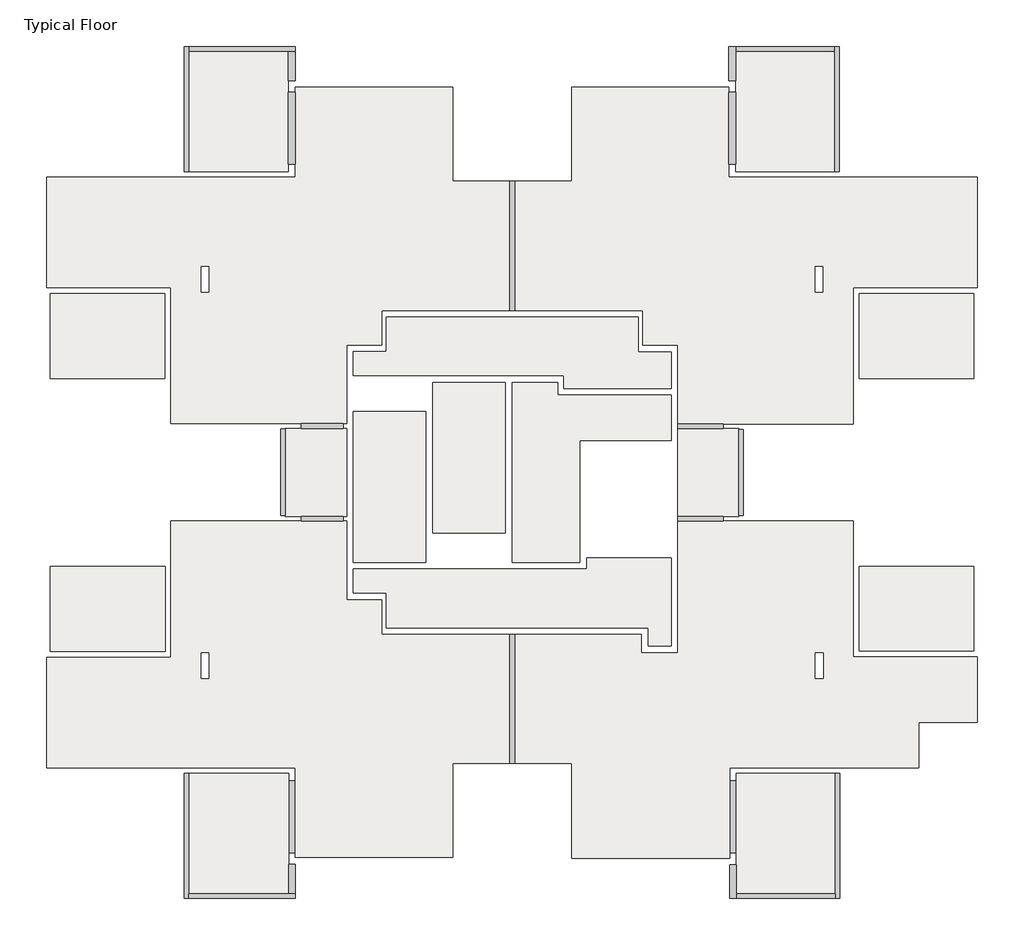
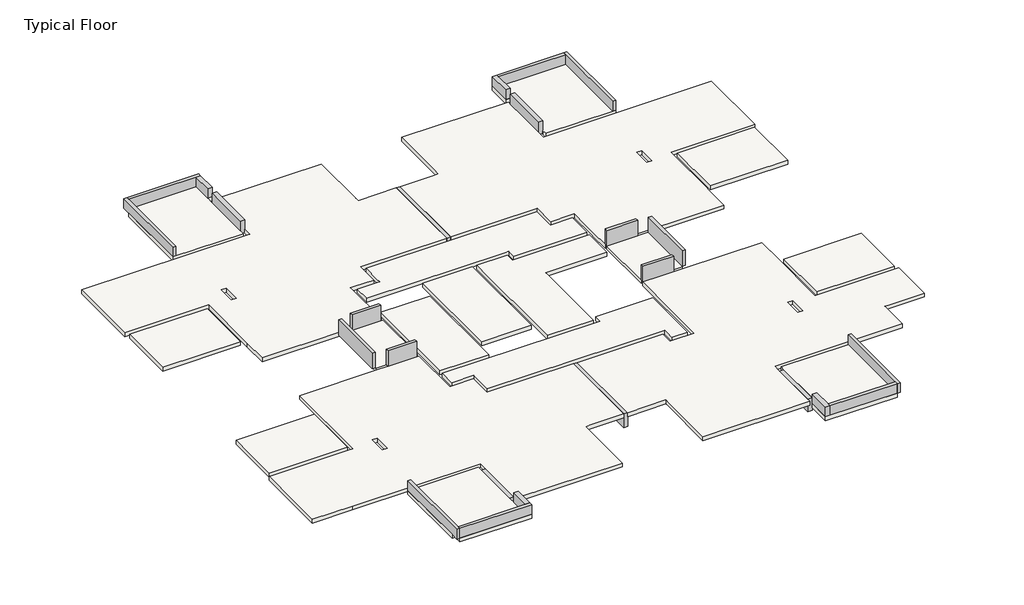
# One storey: 24 beams, 19 slabs.
# Revit data of these elements (continued)
# Element 21 (IfcBeam, "Concrete Rectengular Beam : 22/65") (continued)
#   Mark = "B21"
#   SOFiSTiK_AMG_Comments = ""
#   SOFiSTiK_AMG_Scheduled = yes
#   SOFiSTiK_AMG_Adjusted = yes
#   Structural Material = Concrete
#   Phase Created = New Construction
#   Materials on its faces: "Concrete"
# Element 22 (IfcBeam, "Concrete Rectengular Beam : 22/65")
#   Comments = ""
#   Mark = "B22"
#   SOFiSTiK_AMG_Comments = ""
#   SOFiSTiK_AMG_Scheduled = yes
#   SOFiSTiK_AMG_Adjusted = yes
#   Structural Material = Concrete
#   Phase Created = New Construction
#   Materials on its faces: "Concrete"
# Element 23 (IfcBeam, "Concrete Rectengular Beam : 22/65")
#   Comments = ""
#   Mark = "B23"
#   SOFiSTiK_AMG_Comments = ""
#   SOFiSTiK_AMG_Scheduled = yes
#   SOFiSTiK_AMG_Adjusted = yes
#   Structural Material = Concrete
#   Phase Created = New Construction
#   Materials on its faces: "Concrete"
# Element 24 (IfcBeam, "Concrete Rectengular Beam : 22/65")
#   Comments = ""
#   Mark = "B24"
#   SOFiSTiK_AMG_Comments = ""
#   SOFiSTiK_AMG_Scheduled = yes
#   SOFiSTiK_AMG_Adjusted = yes
#   Structural Material = Concrete
#   Phase Created = New Construction
#   Materials on its faces: "Concrete"
# Element 25 (IfcSlab, "15")
#   Mark = "S18"
#   SOFiSTiK_AMG_Comments = ""
#   built-in parameter 1001955 = 3.14159 (stored number, unit not read)
#   Height Offset From Level = 0 cm
#   built-in parameter 1001954 = 1
#   SOFiSTiK_AMG_Scheduled = yes
#   SOFiSTiK_AMG_Adjusted = yes
#   Phase Created = New Construction
#   Materials on its faces: "Concrete"
# Element 26 (IfcSlab, "15")
#   Mark = "S19"
#   SOFiSTiK_AMG_Comments = ""
#   Height Offset From Level = 0 cm
#   built-in parameter 1001954 = 1
#   SOFiSTiK_AMG_Scheduled = yes
#   SOFiSTiK_AMG_Adjusted = yes
#   Phase Created = New Construction
#   Materials on its faces: "Concrete"
# Element 27 (IfcSlab, "20")
#   Mark = "S1"
#   SOFiSTiK_AMG_Comments = ""
#   Height Offset From Level = 0 cm
#   built-in parameter 1001954 = 1
#   SOFiSTiK_AMG_Scheduled = yes
#   SOFiSTiK_AMG_Adjusted = yes
#   Phase Created = New Construction
#   Materials on its faces: "Concrete"
# Element 28 (IfcSlab, "20")
#   Mark = "S2"
#   SOFiSTiK_AMG_Comments = ""
#   Height Offset From Level = 0 cm
#   built-in parameter 1001954 = 1
#   SOFiSTiK_AMG_Scheduled = yes
#   SOFiSTiK_AMG_Adjusted = yes
#   Phase Created = New Construction
#   Materials on its faces: "Concrete"
# Element 29 (IfcSlab, "20")
#   Mark = "S3"
#   SOFiSTiK_AMG_Comments = ""
#   Height Offset From Level = 0 cm
#   built-in parameter 1001954 = 1
#   SOFiSTiK_AMG_Scheduled = yes
#   SOFiSTiK_AMG_Adjusted = yes
#   Phase Created = New Construction
#   Materials on its faces: "Concrete"
# Element 30 (IfcSlab, "20")
#   Mark = "S4"
#   SOFiSTiK_AMG_Comments = ""
#   Height Offset From Level = 0 cm
#   built-in parameter 1001954 = 1
#   SOFiSTiK_AMG_Scheduled = yes
#   SOFiSTiK_AMG_Adjusted = yes
#   Phase Created = New Construction
#   Materials on its faces: "Concrete"
# Element 31 (IfcSlab, "20")
#   Mark = "S5"
#   SOFiSTiK_AMG_Comments = ""
#   Height Offset From Level = 0 cm
#   built-in parameter 1001954 = 1
#   SOFiSTiK_AMG_Scheduled = yes
#   SOFiSTiK_AMG_Adjusted = yes
#   Phase Created = New Construction
#   Materials on its faces: "Concrete"
# Element 32 (IfcSlab, "20")
#   Mark = "S6"
#   SOFiSTiK_AMG_Comments = ""
#   Height Offset From Level = 0 cm
#   built-in parameter 1001954 = 1
#   SOFiSTiK_AMG_Scheduled = yes
#   SOFiSTiK_AMG_Adjusted = yes
#   Phase Created = New Construction
#   Materials on its faces: "Concrete"
# Element 33 (IfcSlab, "20")
#   Mark = "S7"
#   SOFiSTiK_AMG_Comments = ""
#   Height Offset From Level = 0 cm
#   built-in parameter 1001954 = 1
#   SOFiSTiK_AMG_Scheduled = yes
#   SOFiSTiK_AMG_Adjusted = yes
#   Phase Created = New Construction
#   Materials on its faces: "Concrete"
# Element 34 (IfcSlab, "20")
#   Mark = "S8"
#   SOFiSTiK_AMG_Comments = ""
#   Height Offset From Level = 0 cm
#   built-in parameter 1001954 = 1
#   SOFiSTiK_AMG_Scheduled = yes
#   SOFiSTiK_AMG_Adjusted = yes
#   Phase Created = New Construction
#   Materials on its faces: "Concrete"
# Element 35 (IfcSlab, "20")
#   Mark = "S9"
#   SOFiSTiK_AMG_Comments = ""
#   Height Offset From Level = 0 cm
#   built-in parameter 1001954 = 1
#   SOFiSTiK_AMG_Scheduled = yes
#   SOFiSTiK_AMG_Adjusted = yes
#   Phase Created = New Construction
#   Materials on its faces: "Concrete"
# Element 36 (IfcSlab, "20")
#   Mark = "S10"
#   SOFiSTiK_AMG_Comments = ""
#   built-in parameter 1001955 = 3.14159 (stored number, unit not read)
#   Height Offset From Level = 0 cm
#   built-in parameter 1001954 = 1
#   SOFiSTiK_AMG_Scheduled = yes
#   SOFiSTiK_AMG_Adjusted = yes
#   Phase Created = New Construction
#   Materials on its faces: "Concrete"
# Element 37 (IfcSlab, "20")
#   Mark = "S11"
#   SOFiSTiK_AMG_Comments = ""
#   Height Offset From Level = 0 cm
#   built-in parameter 1001954 = 1
#   SOFiSTiK_AMG_Scheduled = yes
#   SOFiSTiK_AMG_Adjusted = yes
#   Phase Created = New Construction
#   Materials on its faces: "Concrete"
# Element 38 (IfcSlab, "20")
#   Mark = "S12"
#   SOFiSTiK_AMG_Comments = ""
#   Height Offset From Level = 0 cm
#   built-in parameter 1001954 = 1
#   SOFiSTiK_AMG_Scheduled = yes
#   SOFiSTiK_AMG_Adjusted = yes
#   Phase Created = New Construction
#   Materials on its faces: "Concrete"
# Element 39 (IfcSlab, "20")
#   Mark = "S13"
#   SOFiSTiK_AMG_Comments = ""
#   Height Offset From Level = 0 cm
#   built-in parameter 1001954 = 1
#   SOFiSTiK_AMG_Scheduled = yes
#   SOFiSTiK_AMG_Adjusted = yes
#   Phase Created = New Construction
#   Materials on its faces: "Concrete"
# Element 40 (IfcSlab, "20")
#   Mark = "S14"
#   SOFiSTiK_AMG_Comments = ""
#   Height Offset From Level = 0 cm
#   built-in parameter 1001954 = 1
#   SOFiSTiK_AMG_Scheduled = yes
#   SOFiSTiK_AMG_Adjusted = yes
#   Phase Created = New Construction
#   Materials on its faces: "Concrete"
# Element 41 (IfcSlab, "20")
#   Mark = "S15"
#   SOFiSTiK_AMG_Comments = ""
#   Height Offset From Level = 0 cm
#   built-in parameter 1001954 = 1
#   SOFiSTiK_AMG_Scheduled = yes
#   SOFiSTiK_AMG_Adjusted = yes
#   Phase Created = New Construction
#   Materials on its faces: "Concrete"
# Element 42 (IfcSlab, "20")
#   Mark = "S16"
#   SOFiSTiK_AMG_Comments = ""
#   Height Offset From Level = 0 cm
#   built-in parameter 1001954 = 1
#   SOFiSTiK_AMG_Scheduled = yes
#   SOFiSTiK_AMG_Adjusted = yes
#   Phase Created = New Construction
#   Materials on its faces: "Concrete"
# Element 43 (IfcSlab, "20")
#   Mark = "S17"
#   SOFiSTiK_AMG_Comments = ""
#   built-in parameter 1001955 = 1.5708 (stored number, unit not read)
#   Height Offset From Level = 0 cm
#   built-in parameter 1001954 = 1
#   SOFiSTiK_AMG_Scheduled = yes
#   SOFiSTiK_AMG_Adjusted = yes
#   Phase Created = New Construction
#   Materials on its faces: "Concrete"
# Materials
#   "Concrete, Cast-in-Place - B30": class "Concrete", colour RGB 192 192 192, transparency 0, Keynote = "01000", Description = "Cast-in-place concrete", Cost = 0
#   "Concrete": class "Concrete", colour RGB 192 192 192, transparency 0, Keynote = "01000", Description = "Cast-in-place concrete", Cost = 0
